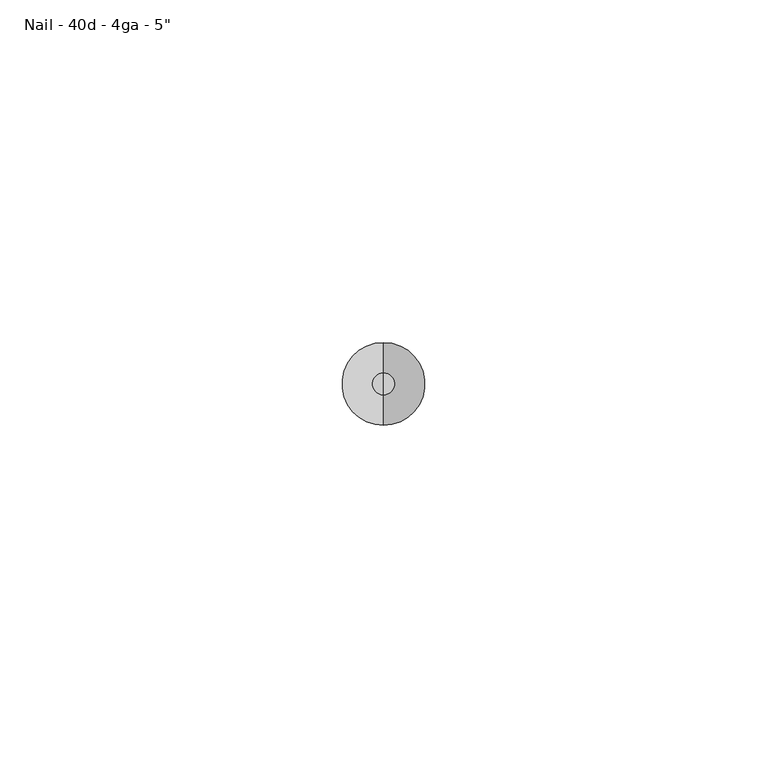
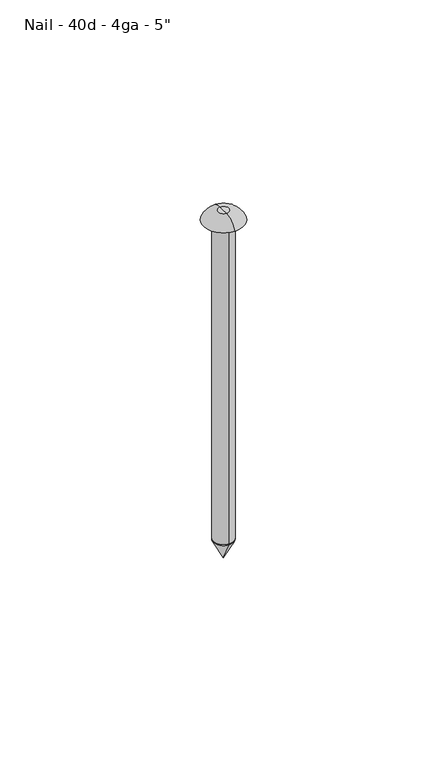
"""IFC4 building model written with IfcOpenShell, lengths in millimetres: fastener geometry."""

import ifcopenshell
import ifcopenshell.guid

model = None  # the IFC model being written
_history = None  # IfcOwnerHistory: only IFC2X3 demands one
_inside = {}  # id of a spatial element -> (the spatial element, [elements in it])
_under = {}  # id of a project, library or spatial element -> (it, [spatial elements below it])
_declared = {}  # id of a project -> (the project, [libraries it declares])
_typed = {}  # id of a type object -> (the type object, [elements of that type])
_made_of = {}  # id of a material, layer set ... -> (it, [elements and type objects made of it])


def new_model(schema):
    """Start an empty IFC model of exactly this schema.

    Asked for "IFC4X3", IfcOpenShell would pick the latest addendum, in which some entities
    have other attributes; the version numbers below select the first issue.
    IFC2X3 requires an IfcOwnerHistory on every rooted entity: one is made here for all.
    """
    global model, _history
    if schema == "IFC4X3":
        model = ifcopenshell.file(schema_version=(4, 3, 0, 0))
    else:
        model = ifcopenshell.file(schema=schema)
    _inside.clear()
    _under.clear()
    _declared.clear()
    _typed.clear()
    _made_of.clear()
    _history = None
    if model.schema == "IFC2X3":
        org = make("IfcOrganization", Name="unknown")
        user = make(
            "IfcPersonAndOrganization",
            ThePerson=make("IfcPerson", FamilyName="unknown"),
            TheOrganization=org,
        )
        app = make(
            "IfcApplication",
            ApplicationDeveloper=org,
            Version="unknown",
            ApplicationFullName="unknown",
            ApplicationIdentifier="unknown",
        )
        _history = make(
            "IfcOwnerHistory",
            OwningUser=user,
            OwningApplication=app,
            ChangeAction="ADDED",
            CreationDate=0,
        )
    return model


def make(cls, **values):
    """One entity of the class cls with the attributes given. An attribute that is None is left unset."""
    return model.create_entity(
        cls, **{name: value for name, value in values.items() if value is not None}
    )


def rooted(cls, **values):
    """An entity with a GlobalId (a new one), such as an element, a storey or a relation."""
    return make(cls, GlobalId=ifcopenshell.guid.new(), OwnerHistory=_history, **values)


def si_unit(unit_type, name, prefix=None):
    """IfcSIUnit, for example si_unit("LENGTHUNIT", "METRE", prefix="MILLI")."""
    return make("IfcSIUnit", UnitType=unit_type, Prefix=prefix, Name=name)


def assignment(units):
    """IfcUnitAssignment: the units of a project."""
    return None if units is None else make("IfcUnitAssignment", Units=units)


def point(xyz):
    """IfcCartesianPoint."""
    return None if xyz is None else make("IfcCartesianPoint", Coordinates=xyz)


def direction(xyz):
    """IfcDirection."""
    return None if xyz is None else make("IfcDirection", DirectionRatios=xyz)


def frame(location, z_axis=None, x_axis=None):
    """IfcAxis2Placement3D, a coordinate frame: its origin and axes. An axis left out is left unset."""
    return make(
        "IfcAxis2Placement3D",
        Location=point(location),
        Axis=direction(z_axis),
        RefDirection=direction(x_axis),
    )


def frame_2d(location, x_axis=None):
    """IfcAxis2Placement2D, a coordinate frame in the plane: its origin and x axis."""
    return make(
        "IfcAxis2Placement2D", Location=point(location), RefDirection=direction(x_axis)
    )


def origin():
    """The frame at (0, 0, 0) with its axes left unset."""
    return frame((0.0, 0.0, 0.0))


def origin_2d():
    """The frame at (0, 0) in the plane with its x axis left unset."""
    return frame_2d((0.0, 0.0))


def place(relative_to, where):
    """IfcLocalPlacement: puts the frame where relative to a parent placement (None: the world)."""
    return make(
        "IfcLocalPlacement", PlacementRelTo=relative_to, RelativePlacement=where
    )


def context(
    kind, dimensions, precision=None, world=None, true_north=None, identifier=None
):
    """IfcGeometricRepresentationContext, for example the 3D "Model" context."""
    return make(
        "IfcGeometricRepresentationContext",
        ContextIdentifier=identifier,
        ContextType=kind,
        CoordinateSpaceDimension=dimensions,
        Precision=precision,
        WorldCoordinateSystem=world,
        TrueNorth=true_north,
    )


def project(units=None, contexts=None):
    """IfcProject with its units and contexts."""
    return rooted(
        "IfcProject",
        Name="project",
        RepresentationContexts=contexts,
        UnitsInContext=assignment(units),
    )


def spatial(cls, under=None, at=None, **own):
    """A site, building, storey or space (cls), placed at a placement, below another one or the project."""
    s = rooted(cls, ObjectPlacement=at, **own)
    if under is not None:
        _under.setdefault(under.id(), (under, []))[1].append(s)
    return s


def polyline(points):
    """IfcPolyline through the points."""
    return make("IfcPolyline", Points=[point(p) for p in points])


def circle_curve(where, radius):
    """IfcCircle in the frame where."""
    return make("IfcCircle", Position=where, Radius=radius)


def ellipse_curve(where, semi_axis1, semi_axis2):
    """IfcEllipse in the frame where."""
    return make(
        "IfcEllipse", Position=where, SemiAxis1=semi_axis1, SemiAxis2=semi_axis2
    )


def trimmed(basis, trim1, trim2, sense, master):
    """IfcTrimmedCurve: the piece of a basis curve between two trims."""
    return make(
        "IfcTrimmedCurve",
        BasisCurve=basis,
        Trim1=trim1,
        Trim2=trim2,
        SenseAgreement=sense,
        MasterRepresentation=master,
    )


def segment(curve, same_sense, transition):
    """IfcCompositeCurveSegment."""
    return make(
        "IfcCompositeCurveSegment",
        Transition=transition,
        SameSense=same_sense,
        ParentCurve=curve,
    )


def composite_curve(segments, self_intersect=None):
    """IfcCompositeCurve: segments joined end to end."""
    return make("IfcCompositeCurve", Segments=segments, SelfIntersect=self_intersect)


def outline(outer, holes=None, kind="AREA"):
    """IfcArbitraryClosedProfileDef: a profile drawn as a closed curve; with holes, ...WithVoids."""
    if holes is None:
        return make("IfcArbitraryClosedProfileDef", ProfileType=kind, OuterCurve=outer)
    return make(
        "IfcArbitraryProfileDefWithVoids",
        ProfileType=kind,
        OuterCurve=outer,
        InnerCurves=holes,
    )


def extrude(swept, where, along, depth):
    """IfcExtrudedAreaSolid: the profile swept, set in the frame where, extruded along a direction by depth."""
    return make(
        "IfcExtrudedAreaSolid",
        SweptArea=swept,
        Position=where,
        ExtrudedDirection=direction(along),
        Depth=depth,
    )


def shape(context_of_items, identifier, shape_type, items):
    """IfcShapeRepresentation: the items that make up one representation, for example the "Body"."""
    return make(
        "IfcShapeRepresentation",
        ContextOfItems=context_of_items,
        RepresentationIdentifier=identifier,
        RepresentationType=shape_type,
        Items=items,
    )


def source(mapping_origin, context_of_items, identifier, shape_type, items):
    """IfcRepresentationMap: a shape defined once, which mapped items show again and again."""
    return make(
        "IfcRepresentationMap",
        MappingOrigin=mapping_origin,
        MappedRepresentation=shape(context_of_items, identifier, shape_type, items),
    )


def transform(
    local_origin,
    x_axis=None,
    y_axis=None,
    z_axis=None,
    scale=None,
    scale2=None,
    scale3=None,
    uniform=True,
):
    """IfcCartesianTransformationOperator3D, or its non-uniform kind. x_axis, y_axis, z_axis: its Axis1, 2, 3."""
    if uniform:
        return make(
            "IfcCartesianTransformationOperator3D",
            Axis1=direction(x_axis),
            Axis2=direction(y_axis),
            LocalOrigin=point(local_origin),
            Scale=scale,
            Axis3=direction(z_axis),
        )
    return make(
        "IfcCartesianTransformationOperator3DnonUniform",
        Axis1=direction(x_axis),
        Axis2=direction(y_axis),
        LocalOrigin=point(local_origin),
        Scale=scale,
        Axis3=direction(z_axis),
        Scale2=scale2,
        Scale3=scale3,
    )


def mapped(mapping_source, mapping_target):
    """IfcMappedItem: shows the shape of a source again, moved by a transform."""
    return make(
        "IfcMappedItem", MappingSource=mapping_source, MappingTarget=mapping_target
    )


def made_of(thing, what):
    """Note that an element or type object is made of a material, layer set ...; save() writes the relation."""
    if what is not None:
        _made_of.setdefault(what.id(), (what, []))[1].append(thing)
    return thing


def element(
    cls,
    number,
    at=None,
    inside=None,
    cuts=None,
    type_object=None,
    material=None,
    context=None,
    identifier="Body",
    shape_type=None,
    held_by="IfcProductDefinitionShape",
    body=None,
    shapes=None,
    **own,
):
    """One element of the class cls, such as IfcWall. Its Tag is "e" and its number.

    at: its placement. inside: the storey or other place that contains it. cuts: it is an
    opening in that element (IfcRelVoidsElement). A single representation is given by context,
    identifier, shape_type and body (its items); several are given by shapes. held_by: the class
    of the entity that holds the representations. save() writes the other relations.
    """
    e = rooted(cls, Tag="e%d" % number, ObjectPlacement=at, **own)
    if body is not None:
        shapes = [shape(context, identifier, shape_type, body)]
    if shapes is not None:
        e.Representation = make(held_by, Representations=shapes)
    if inside is not None:
        _inside.setdefault(inside.id(), (inside, []))[1].append(e)
    if cuts is not None:
        rooted(
            "IfcRelVoidsElement", RelatingBuildingElement=cuts, RelatedOpeningElement=e
        )
    if type_object is not None:
        _typed.setdefault(type_object.id(), (type_object, []))[1].append(e)
    return made_of(e, material)


def aggregate(whole, parts):
    """IfcRelAggregates: a whole, such as a stair, and the parts it consists of."""
    return rooted("IfcRelAggregates", RelatingObject=whole, RelatedObjects=parts)


def save(model, path):
    """Write the relations noted so far, then the file.

    IfcRelAggregates (storeys below a building ...), IfcRelContainedInSpatialStructure (elements
    in a storey), IfcRelDefinesByType, IfcRelAssociatesMaterial and IfcRelDeclares: one each for
    every whole, place, type object, material and project.
    """
    for whole, parts in _under.values():
        aggregate(whole, parts)
    for where, things in _inside.values():
        rooted(
            "IfcRelContainedInSpatialStructure",
            RelatedElements=things,
            RelatingStructure=where,
        )
    for kind, things in _typed.values():
        rooted("IfcRelDefinesByType", RelatedObjects=things, RelatingType=kind)
    for what, things in _made_of.values():
        rooted("IfcRelAssociatesMaterial", RelatedObjects=things, RelatingMaterial=what)
    for by, libraries in _declared.values():
        rooted("IfcRelDeclares", RelatingContext=by, RelatedDefinitions=libraries)
    model.write(path)


def plane_surface(at):
    """IfcPlane: the flat surface through the origin of the frame at, square to its z axis."""
    return make("IfcPlane", Position=at)


def revolved_surface(curve, axis_point, axis_direction):
    """IfcSurfaceOfRevolution: the curve turned about the line through axis_point along axis_direction."""
    return make(
        "IfcSurfaceOfRevolution",
        SweptCurve=make("IfcArbitraryOpenProfileDef", ProfileType="CURVE", Curve=curve),
        AxisPosition=make("IfcAxis1Placement", Location=point(axis_point), Axis=direction(axis_direction)),
    )


def advanced_brep(points, edges, surfaces, faces):
    """IfcAdvancedBrep: a solid bounded by faces that lie on surfaces and meet in shared edges.

    An edge is (start, end): straight between two places in points (the first is 0);
    or (start, end, curve); or (start, end, curve, False) where it runs against its curve.
    A face is (place in surfaces, loops), or (place, loops, False) where it looks against
    its surface's normal. A loop lists edges by number (the first is 1), with a minus sign
    where the edge is run from its end to its start. The first loop is the outer one.
    """
    corners = [point(p) for p in points]
    vertices = [make("IfcVertexPoint", VertexGeometry=c) for c in corners]
    made = []
    for start, end, *more in edges:
        made.append(
            make(
                "IfcEdgeCurve",
                EdgeStart=vertices[start],
                EdgeEnd=vertices[end],
                EdgeGeometry=more[0] if more else make("IfcPolyline", Points=[corners[start], corners[end]]),
                SameSense=more[1] if len(more) > 1 else True,
            )
        )
    hull = []
    for where, loops, *sense in faces:
        bounds = []
        for j, loop in enumerate(loops):
            ring = [make("IfcOrientedEdge", EdgeElement=made[abs(k) - 1], Orientation=k > 0) for k in loop]
            bounds.append(
                make(
                    "IfcFaceOuterBound" if j == 0 else "IfcFaceBound",
                    Bound=make("IfcEdgeLoop", EdgeList=ring),
                    Orientation=True,
                )
            )
        hull.append(make("IfcAdvancedFace", Bounds=bounds, FaceSurface=surfaces[where], SameSense=sense[0] if sense else True))
    return make("IfcAdvancedBrep", Outer=make("IfcClosedShell", CfsFaces=hull))


def fastener_0606e984(model_context):
    return source(origin(), model_context, "Body", "SolidModel", [
        advanced_brep(
        [(0.0, -3.0226, -101.6), (0.0, 3.0226, -101.6), (0.0, 0.0, -101.6), (0.0, 0.0, -107.6452)],
        [
            (0, 1, circle_curve(frame((0.0, 0.0, -101.6), z_axis=(0.0, 0.0, 1.0), x_axis=(0.0, 1.0, 0.0)), 3.0226)),
            (1, 2),
            (2, 0),
            (1, 0, circle_curve(frame((0.0, 0.0, -101.6), z_axis=(0.0, 0.0, 1.0), x_axis=(0.0, 1.0, 0.0)), 3.0226)),
            (3, 1),
            (0, 3),
        ],
        [
            plane_surface(frame((0.0, 0.0, -101.6), z_axis=(0.0, 0.0, 1.0), x_axis=(0.0, 1.0, 0.0))),
            revolved_surface(polyline([(0.0, 3.0226, -101.6), (0.0, 0.0, -107.6452)]), (0.0, 0.0, -103.0840259), (0.0, 0.0, -1.0)),
        ],
        [
            (0, [[1, 2, 3]]),
            (0, [[4, -3, -2]]),
            (1, [[5, -1, 6]]),
            (1, [[-6, -4, -5]]),
        ],
    ),
        advanced_brep(
        [(0.0, 6.0452, 0.0), (0.0, -6.0452, 0.0), (0.0, 0.0, 0.0), (0.0, 0.0, 3.0226), (0.0, -1.5875, 3.0226), (0.0, 1.5875, 3.0226)],
        [
            (0, 1, circle_curve(frame((0.0, 0.0, 0.0), z_axis=(0.0, 0.0, -1.0), x_axis=(0.0, -1.0, 0.0)), 6.0452)),
            (1, 2),
            (2, 0),
            (1, 0, circle_curve(frame((0.0, 0.0, 0.0), z_axis=(0.0, 0.0, -1.0), x_axis=(0.0, -1.0, 0.0)), 6.0452)),
            (3, 4),
            (4, 5, circle_curve(frame((0.0, 0.0, 3.0226), z_axis=(0.0, 0.0, 1.0), x_axis=(0.0, -1.0, 0.0)), 1.5875)),
            (5, 3),
            (5, 4, circle_curve(frame((0.0, 0.0, 3.0226), z_axis=(0.0, 0.0, 1.0), x_axis=(0.0, -1.0, 0.0)), 1.5875)),
            (4, 1, circle_curve(frame((0.0, -1.5875, -1.7757855), z_axis=(1.0, 0.0, 0.0), x_axis=(0.0, -1.0, 0.0)), 4.7983855)),
            (0, 5, circle_curve(frame((0.0, 1.5875, -1.7757855), z_axis=(1.0, 0.0, 0.0), x_axis=(0.0, 1.0, 0.0)), 4.7983855)),
        ],
        [
            plane_surface(frame((0.0, 0.0, 0.0), z_axis=(0.0, 0.0, -1.0), x_axis=(0.0, -1.0, 0.0))),
            plane_surface(frame((0.0, 0.0, 3.0226), z_axis=(0.0, 0.0, 1.0), x_axis=(0.0, -1.0, 0.0))),
            revolved_surface(trimmed(ellipse_curve(frame((0.0, -1.5875, -1.7757855), z_axis=(-1.0, 0.0, 0.0), x_axis=(0.0, -1.0, 0.0)), 4.7983855, 4.7983855), [point((0.0, -6.0452, 0.0))], [point((0.0, -1.5875, 3.0226))], True, "CARTESIAN"), (0.0, 0.0, 1.4840259), (0.0, 0.0, 1.0)),
        ],
        [
            (0, [[1, 2, 3]]),
            (0, [[4, -3, -2]]),
            (1, [[5, 6, 7]]),
            (1, [[-7, 8, -5]]),
            (2, [[-6, 9, -1, 10]]),
            (2, [[-8, -10, -4, -9]]),
        ],
    ),
        extrude(outline(composite_curve([segment(trimmed(circle_curve(origin_2d(), 3.0226), [point((0.0, -3.0226))], [point((0.0, 3.0226))], False, "CARTESIAN"), True, "CONTINUOUS"), segment(trimmed(circle_curve(origin_2d(), 3.0226), [point((0.0, 3.0226))], [point((0.0, -3.0226))], False, "CARTESIAN"), True, "CONTINUOUS")], self_intersect=False)), frame((0.0, 0.0, -101.6), z_axis=(0.0, 0.0, 1.0), x_axis=(1.0, 0.0, 0.0)), (0.0, 0.0, 1.0), 101.6),
    ])


if __name__ == "__main__":
    model = new_model("IFC4")
    model_context = context("Model", 3, world=origin())
    ifc_project = project(units=[si_unit("LENGTHUNIT", "METRE", prefix="MILLI")], contexts=[model_context])
    site = spatial("IfcSite", under=ifc_project)
    building = spatial("IfcBuilding", under=site)
    placement = place(None, origin())
    fastener_shape = fastener_0606e984(model_context)
    element("IfcFastener", 1, ObjectType="060523 - W_P_C - Fastenings - Generic : Nail - 40d - 4ga - 5\"", at=placement, inside=building, context=model_context, shape_type="MappedRepresentation", body=[
        mapped(fastener_shape, transform((0.0, 0.0, 0.0), x_axis=(1.0, 0.0, 0.0), y_axis=(0.0, 1.0, 0.0), z_axis=(0.0, 0.0, 1.0))),
    ])
    save(model, "model.ifc")

# Revit data of these elements
# Type "060523 - W_P_C - Fastenings - Generic : Nail - 40d - 4ga - 5\""
#   Washer_Thickness = 0' - 0.00333"
#   Washer Radius = 0' - 0.129"
#   Washer Offset - Head = 0' - 0"
#   Washer Offset = 0' - 0"
#   Thickness_of_Substrate [instance default] = 0' - 1"
#   Side = 0' - 0 37/64"
#   Radius = 0' - 0.119"
#   Length [instance default] = 0' - 5"
#   Head Size = 0' - 1"
#   Head Radius = 0' - 0 1/2"
#   Head Height = 0' - 0.01"
#   Double Diameter = 0' - 0.476"
#   Diameter = 0' - 0.238"
#   Default Elevation = 4' - 0"
#   Washer_Nut_Visibility = no
#   Washer_Head_Visibility = no
#   Round_Head_Visibility = yes
#   Point Visibility = yes
#   Nut_Visibility = no
#   Hex_Head_Visiblilty = no
#   Washer Material = none
#   Bolt Material (Size) = AT SILL - FASTENER AT 24" O.C.
# Element 1 (IfcFastener, "060523 - W_P_C - Fastenings - Generic : Nail - 40d - 4ga - 5\"")
#   Length = 0' - 4"
#   Materials on its faces: "AT SILL - FASTENER AT 24\" O.C."
# Materials
#   "AT SILL - FASTENER AT 24\" O.C.": class "Generic", colour RGB 120 120 120, transparency 0, Cost = 0
